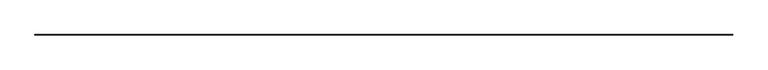
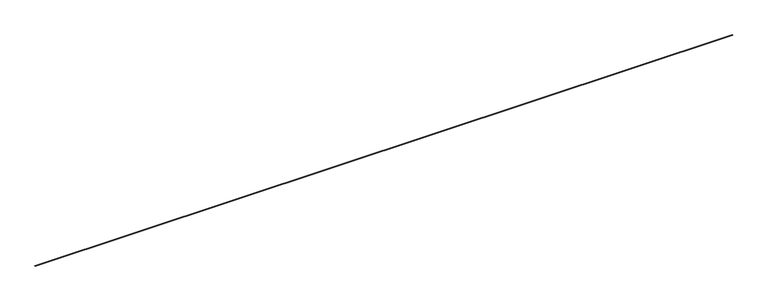
"""IFC4 building model written with IfcOpenShell, lengths in millimetres: proxy geometry, Inner panel:Inner panel:1:Inner panel:1 : Inner panel:Inner panel:300324:2:Inner panel:1:Inner panel:1 : Inner panel:Inner panel:300324:2 : Inner panel:Inner panel:1:Inner panel:1 : Inner panel:Inner panel:300324:300043:10 : Inner panel:Inner panel:1:Inner panel:1 : Inner panel:Inner panel:300324:2:Inner panel:1:Inner panel:1 : Inner panel:Inner panel:300324:2 : Inner panel:Inner panel:1:Inner panel:1 : Inner panel:Inner panel:300324:300043:308120."""

from ifc_helpers import new_model, si_unit, frame, origin, place, context, project, spatial, polyline, outline, extrude, source, transform, mapped, element, save


def generic_models_ceca976f(model_context):
    return source(origin(), model_context, "Body", "SweptSolid", [
        extrude(outline(polyline([(-568255.3503852, 8762.7000209), (-568256.9365089, 8800.7669909), (-568218.8695388, 8802.3531147), (-568217.2834151, 8764.2861446), (-568255.3503852, 8762.7000209)]), holes=[polyline([(-568253.0703323, 8765.1783392), (-568219.7617335, 8766.5661975), (-568221.1495917, 8799.8747963), (-568254.4581906, 8798.4869381), (-568253.0703323, 8765.1783392)])]), frame((579104.5117239, 0.0, 0.0), z_axis=(1.0, 0.0, 0.0), x_axis=(0.0, 1.0, 0.0)), (0.0, 0.0, 1.0), 88442.8),
    ])


if __name__ == "__main__":
    model = new_model("IFC4")
    model_context = context("Model", 3, world=origin())
    ifc_project = project(units=[si_unit("LENGTHUNIT", "METRE", prefix="MILLI")], contexts=[model_context])
    site = spatial("IfcSite", under=ifc_project)
    building = spatial("IfcBuilding", under=site)
    placement = place(None, origin())
    generic_models_shape = generic_models_ceca976f(model_context)
    element("IfcBuildingElementProxy", 1, Name="Inner panel:Inner panel:1:Inner panel:1 : Inner panel:Inner panel:300324:2:Inner panel:1:Inner panel:1 : Inner panel:Inner panel:300324:2 : Inner panel:Inner panel:1:Inner panel:1 : Inner panel:Inner panel:300324:300043:10 : Inner panel:Inner panel:1:Inner panel:1 : Inner panel:Inner panel:300324:2:Inner panel:1:Inner panel:1 : Inner panel:Inner panel:300324:2 : Inner panel:Inner panel:1:Inner panel:1 : Inner panel:Inner panel:300324:300043:308120", ObjectType="Inner panel:Inner panel:1:Inner panel:1 : Inner panel:Inner panel:300324:2:Inner panel:1:Inner panel:1 : Inner panel:Inner panel:300324:2 : Inner panel:Inner panel:1:Inner panel:1 : Inner panel:Inner panel:300324:300043:10 : Inner panel:Inner panel:1:Inner panel:1 : Inner panel:Inner panel:300324:2:Inner panel:1:Inner panel:1 : Inner panel:Inner panel:300324:2 : Inner panel:Inner panel:1:Inner panel:1 : Inner panel:Inner panel:300324:300043:308120", at=placement, inside=building, context=model_context, shape_type="MappedRepresentation", body=[
        mapped(generic_models_shape, transform((0.0, 0.0, 0.0), x_axis=(1.0, 0.0, 0.0), y_axis=(0.0, 1.0, 0.0), z_axis=(0.0, 0.0, 1.0))),
    ])
    save(model, "model.ifc")

# Revit data of these elements
# Type "Inner panel:Inner panel:1:Inner panel:1 : Inner panel:Inner panel:300324:2:Inner panel:1:Inner panel:1 : Inner panel:Inner panel:300324:2 : Inner panel:Inner panel:1:Inner panel:1 : Inner panel:Inner panel:300324:300043:10 : Inner panel:Inner panel:1:Inner panel:1 : Inner panel:Inner panel:300324:2:Inner panel:1:Inner panel:1 : Inner panel:Inner panel:300324:2 : Inner panel:Inner panel:1:Inner panel:1 : Inner panel:Inner panel:300324:300043:308120"
#   NameOverride = "Inner panel:Inner panel:1:Inner panel:1 : Inner panel:Inner panel:300324:2:Inner panel:1:Inner panel:1 : Inner panel:Inner panel:300324:2 : Inner panel:Inner panel:1:Inner panel:1 : Inner panel:Inner panel:300324:300043:308120"
#   ObjectTypeOverride = "Inner panel:1:Inner panel:1 : Inner panel:Inner panel:300324:2 : Inner panel:Inner panel:1:Inner panel:1 : Inner panel:Inner panel:300324:300043"
#   Reference = "Inner panel"
#   Tag = "308120"
# Element 1 (IfcBuildingElementProxy, "Inner panel:Inner panel:1:Inner panel:1 : Inner panel:Inner panel:300324:2:Inner panel:1:Inner panel:1 : Inner panel:Inner panel:300324:2 : Inner panel:Inner panel:1:Inner panel:1 : Inner panel:Inner panel:300324:300043:10 : Inner panel:Inner panel:1:Inner panel:1 : Inner panel:Inner panel:300324:2:Inner panel:1:Inner panel:1 : Inner panel:Inner panel:300324:2 : Inner panel:Inner panel:1:Inner panel:1 : Inner panel:Inner panel:300324:300043:308120")
#   Materials on its faces: "1 1/2\" X 1 1/2\" x 1/8\" ALUM. TUBE (6061-T6) - (2) #16 WOOD SCREWS WITH 2.5\" EMBED AT EACH GLULAM - (1) SCREW AT ENDS"
# Materials
#   "1 1/2\" X 1 1/2\" x 1/8\" ALUM. TUBE (6061-T6) - (2) #16 WOOD SCREWS WITH 2.5\" EMBED AT EACH GLULAM - (1) SCREW AT ENDS": class "Unassigned", colour RGB 202 201 200, transparency 0, Cost = 0
